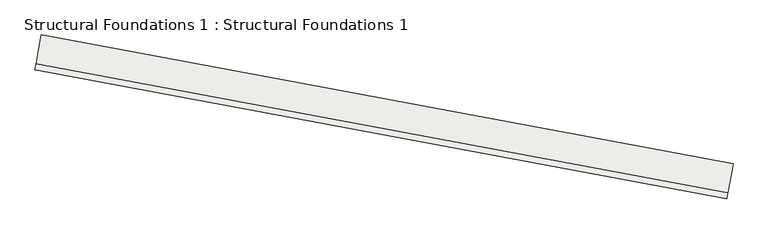
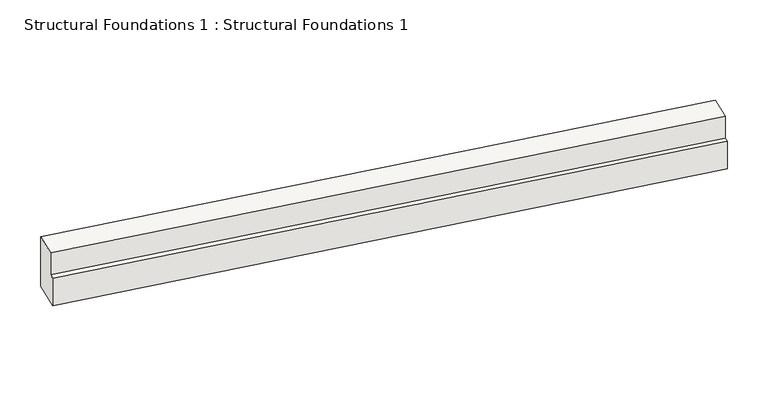
"""IFC4 building model written with IfcOpenShell, lengths in millimetres: slab geometry, Structural Foundations 1 : Structural Foundations 1."""

from ifc_helpers import new_model, si_unit, frame, origin, place, context, project, spatial, polyline, outline, extrude, source, transform, mapped, element, save


def structural_foundations_1_structural_foundations_1_fabcf75b(model_context):
    return source(origin(), model_context, "Body", "SweptSolid", [
        extrude(outline(polyline([(587.375, 0.0), (587.375, -527.05), (711.2, -527.05), (711.2, -1187.45), (0.0, -1187.45), (0.0, -527.05), (0.0, 0.0), (587.375, 0.0)])), frame((-60378.1813443, 38575.8809234, 9239.25), z_axis=(-0.9830688624224048, 0.1832364912770354, 0.0), x_axis=(-0.1832364912770354, -0.9830688624224048, 0.0)), (0.0, 0.0, 1.0), 14097.0),
    ])


if __name__ == "__main__":
    model = new_model("IFC4")
    model_context = context("Model", 3, world=origin())
    ifc_project = project(units=[si_unit("LENGTHUNIT", "METRE", prefix="MILLI")], contexts=[model_context])
    site = spatial("IfcSite", under=ifc_project)
    building = spatial("IfcBuilding", under=site)
    placement = place(None, origin())
    structural_foundations_1_structural_foundations_1_shape = structural_foundations_1_structural_foundations_1_fabcf75b(model_context)
    element("IfcSlab", 1, ObjectType="Structural Foundations 1 : Structural Foundations 1", at=placement, inside=building, context=model_context, shape_type="MappedRepresentation", body=[
        mapped(structural_foundations_1_structural_foundations_1_shape, transform((0.0, 0.0, 0.0), x_axis=(1.0, 0.0, 0.0), y_axis=(0.0, 1.0, 0.0), z_axis=(0.0, 0.0, 1.0))),
    ])
    save(model, "model.ifc")

# Revit data of these elements
# Element 1 (IfcSlab, "Structural Foundations 1 : Structural Foundations 1")
#   Materials on its faces: "16 - Concrete - Cast-in-Place"
# Materials
#   "16 - Concrete - Cast-in-Place": class "Unassigned", colour RGB 192 192 192, transparency 0, Description = "Concrete", Cost = 0
